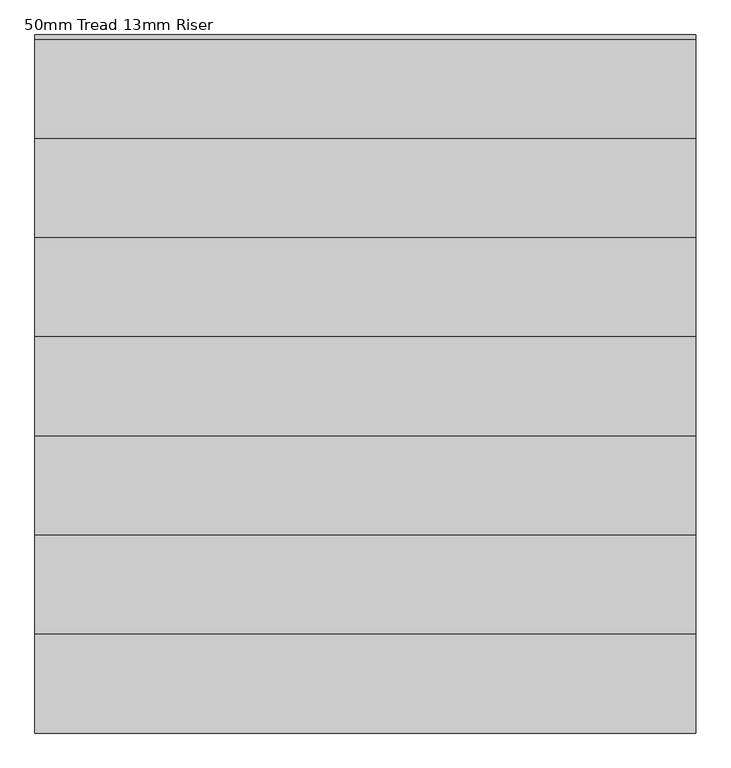
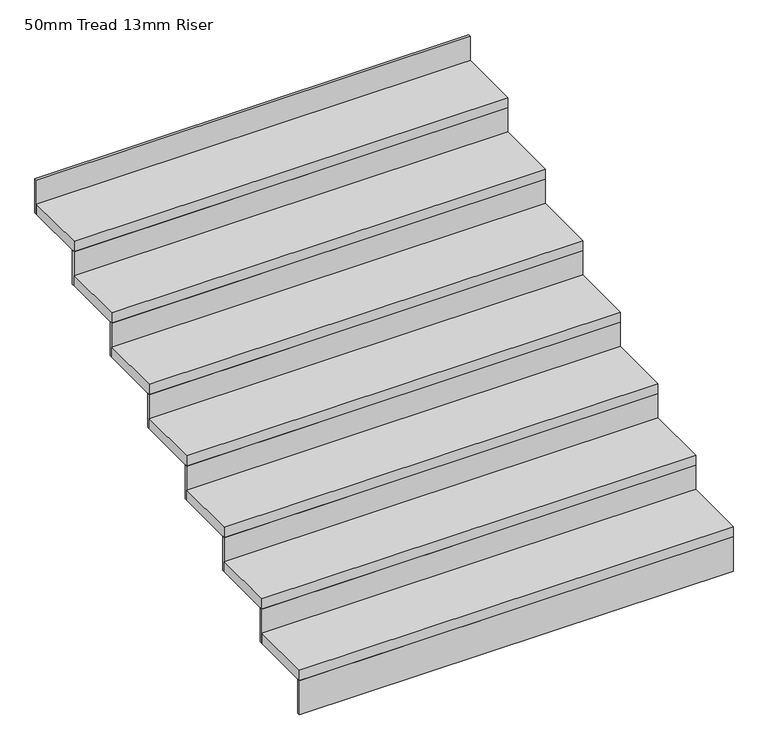
"""IFC4 building model written with IfcOpenShell, lengths in millimetres: stair flight geometry, 50mm Tread 13mm Riser."""

from ifc_helpers import new_model, si_unit, frame, origin, place, context, project, spatial, polyline, outline, extrude, source, transform, mapped, element, save


def stair_flight_50mm_tread_13mm_riser_257646a8(model_context):
    return source(origin(), model_context, "Body", "SweptSolid", [
        extrude(outline(polyline([(14700.0002443, 21382.4999999), (14700.0002443, 21369.9999999), (12700.0002443, 21369.9999999), (12700.0002443, 21382.4999999), (14700.0002443, 21382.4999999)])), frame((0.0, 0.0, 23616.6666667), z_axis=(0.0, 0.0, 1.0), x_axis=(1.0, 0.0, 0.0)), (0.0, 0.0, 1.0), 166.6666667),
        extrude(outline(polyline([(12700.0002443, 21669.9999999), (14700.0002443, 21669.9999999), (14700.0002443, 21369.9999999), (12700.0002443, 21369.9999999), (12700.0002443, 21669.9999999)])), frame((0.0, 0.0, 23783.3333333), z_axis=(0.0, 0.0, 1.0), x_axis=(1.0, 0.0, 0.0)), (0.0, 0.0, 1.0), 50.0),
        extrude(outline(polyline([(14700.0002443, 21682.4999999), (14700.0002443, 21669.9999999), (12700.0002443, 21669.9999999), (12700.0002443, 21682.4999999), (14700.0002443, 21682.4999999)])), frame((0.0, 0.0, 23783.3333333), z_axis=(0.0, 0.0, 1.0), x_axis=(1.0, 0.0, 0.0)), (0.0, 0.0, 1.0), 166.6666667),
        extrude(outline(polyline([(12700.0002443, 21969.9999999), (14700.0002443, 21969.9999999), (14700.0002443, 21669.9999999), (12700.0002443, 21669.9999999), (12700.0002443, 21969.9999999)])), frame((0.0, 0.0, 23950.0), z_axis=(0.0, 0.0, 1.0), x_axis=(1.0, 0.0, 0.0)), (0.0, 0.0, 1.0), 50.0),
        extrude(outline(polyline([(14700.0002443, 21982.4999999), (14700.0002443, 21969.9999999), (12700.0002443, 21969.9999999), (12700.0002443, 21982.4999999), (14700.0002443, 21982.4999999)])), frame((0.0, 0.0, 23950.0), z_axis=(0.0, 0.0, 1.0), x_axis=(1.0, 0.0, 0.0)), (0.0, 0.0, 1.0), 166.6666667),
        extrude(outline(polyline([(12700.0002443, 22269.9999999), (14700.0002443, 22269.9999999), (14700.0002443, 21969.9999999), (12700.0002443, 21969.9999999), (12700.0002443, 22269.9999999)])), frame((0.0, 0.0, 24116.6666667), z_axis=(0.0, 0.0, 1.0), x_axis=(1.0, 0.0, 0.0)), (0.0, 0.0, 1.0), 50.0),
        extrude(outline(polyline([(14700.0002443, 22282.4999999), (14700.0002443, 22269.9999999), (12700.0002443, 22269.9999999), (12700.0002443, 22282.4999999), (14700.0002443, 22282.4999999)])), frame((0.0, 0.0, 24116.6666667), z_axis=(0.0, 0.0, 1.0), x_axis=(1.0, 0.0, 0.0)), (0.0, 0.0, 1.0), 166.6666667),
        extrude(outline(polyline([(12700.0002443, 22569.9999999), (14700.0002443, 22569.9999999), (14700.0002443, 22269.9999999), (12700.0002443, 22269.9999999), (12700.0002443, 22569.9999999)])), frame((0.0, 0.0, 24283.3333333), z_axis=(0.0, 0.0, 1.0), x_axis=(1.0, 0.0, 0.0)), (0.0, 0.0, 1.0), 50.0),
        extrude(outline(polyline([(14700.0002443, 22582.4999999), (14700.0002443, 22569.9999999), (12700.0002443, 22569.9999999), (12700.0002443, 22582.4999999), (14700.0002443, 22582.4999999)])), frame((0.0, 0.0, 24283.3333333), z_axis=(0.0, 0.0, 1.0), x_axis=(1.0, 0.0, 0.0)), (0.0, 0.0, 1.0), 166.6666667),
        extrude(outline(polyline([(12700.0002443, 22869.9999999), (14700.0002443, 22869.9999999), (14700.0002443, 22569.9999999), (12700.0002443, 22569.9999999), (12700.0002443, 22869.9999999)])), frame((0.0, 0.0, 24450.0), z_axis=(0.0, 0.0, 1.0), x_axis=(1.0, 0.0, 0.0)), (0.0, 0.0, 1.0), 50.0),
        extrude(outline(polyline([(14700.0002443, 22882.4999999), (14700.0002443, 22869.9999999), (12700.0002443, 22869.9999999), (12700.0002443, 22882.4999999), (14700.0002443, 22882.4999999)])), frame((0.0, 0.0, 24450.0), z_axis=(0.0, 0.0, 1.0), x_axis=(1.0, 0.0, 0.0)), (0.0, 0.0, 1.0), 166.6666667),
        extrude(outline(polyline([(12700.0002443, 23169.9999999), (14700.0002443, 23169.9999999), (14700.0002443, 22869.9999999), (12700.0002443, 22869.9999999), (12700.0002443, 23169.9999999)])), frame((0.0, 0.0, 24616.6666667), z_axis=(0.0, 0.0, 1.0), x_axis=(1.0, 0.0, 0.0)), (0.0, 0.0, 1.0), 50.0),
        extrude(outline(polyline([(14700.0002443, 23182.4999999), (14700.0002443, 23169.9999999), (12700.0002443, 23169.9999999), (12700.0002443, 23182.4999999), (14700.0002443, 23182.4999999)])), frame((0.0, 0.0, 24616.6666667), z_axis=(0.0, 0.0, 1.0), x_axis=(1.0, 0.0, 0.0)), (0.0, 0.0, 1.0), 166.6666667),
        extrude(outline(polyline([(14700.0002443, 23482.4999999), (14700.0002443, 23469.9999999), (12700.0002443, 23469.9999999), (12700.0002443, 23482.4999999), (14700.0002443, 23482.4999999)])), frame((0.0, 0.0, 24783.3333333), z_axis=(0.0, 0.0, 1.0), x_axis=(1.0, 0.0, 0.0)), (0.0, 0.0, 1.0), 166.6666667),
        extrude(outline(polyline([(12700.0002443, 23469.9999999), (14700.0002443, 23469.9999999), (14700.0002443, 23169.9999999), (12700.0002443, 23169.9999999), (12700.0002443, 23469.9999999)])), frame((0.0, 0.0, 24783.3333333), z_axis=(0.0, 0.0, 1.0), x_axis=(1.0, 0.0, 0.0)), (0.0, 0.0, 1.0), 50.0),
    ])


if __name__ == "__main__":
    model = new_model("IFC4")
    model_context = context("Model", 3, world=origin())
    ifc_project = project(units=[si_unit("LENGTHUNIT", "METRE", prefix="MILLI")], contexts=[model_context])
    site = spatial("IfcSite", under=ifc_project)
    building = spatial("IfcBuilding", under=site)
    placement = place(None, origin())
    stair_flight_50mm_tread_13mm_riser_shape = stair_flight_50mm_tread_13mm_riser_257646a8(model_context)
    element("IfcStairFlight", 1, ObjectType="50mm Tread 13mm Riser", at=placement, inside=building, context=model_context, shape_type="MappedRepresentation", body=[
        mapped(stair_flight_50mm_tread_13mm_riser_shape, transform((0.0, 0.0, 0.0), x_axis=(1.0, 0.0, 0.0), y_axis=(0.0, 1.0, 0.0), z_axis=(0.0, 0.0, 1.0))),
    ])
    save(model, "model.ifc")

# Revit data of these elements
# Project information
#   Project Issue Date = "Issue Date"
#   Project Status = "Project Status"
#   Client Name = "Owner"
#   Project Address = "Enter address here"
#   Project Name = "Project Name"
#   Project Number = "0001"
